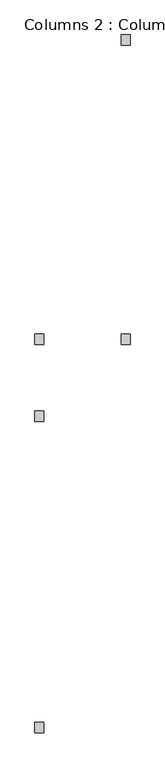
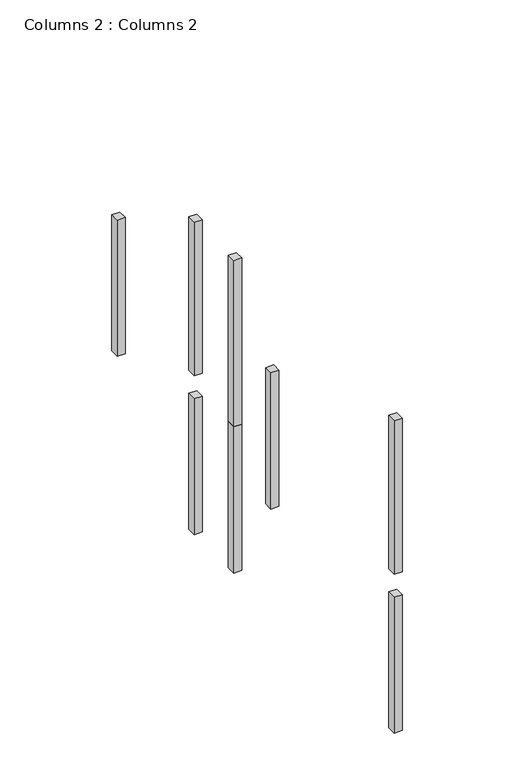
"""IFC4 building model written with IfcOpenShell, lengths in millimetres: column geometry, Columns 2 : Columns 2."""

from ifc_helpers import new_model, si_unit, frame, origin, place, context, project, spatial, polyline, outline, extrude, source, transform, mapped, element, save


def columns_2_columns_2_417d1360(model_context):
    return source(origin(), model_context, "Body", "SweptSolid", [
        extrude(outline(polyline([(31923.0340778, 35213.6207942), (31923.0340778, 35366.0207942), (32053.2090778, 35366.0207942), (32053.2090778, 35213.6207942), (31923.0340778, 35213.6207942)])), frame((0.0, 0.0, 268947.9), z_axis=(0.0, 0.0, 1.0), x_axis=(1.0, 0.0, 0.0)), (0.0, 0.0, 1.0), 2857.5),
        extrude(outline(polyline([(31923.0340778, 36331.2207942), (31923.0340778, 36483.6207942), (32053.2090778, 36483.6207942), (32053.2090778, 36331.2207942), (31923.0340778, 36331.2207942)])), frame((0.0, 0.0, 266414.25), z_axis=(0.0, 0.0, 1.0), x_axis=(1.0, 0.0, 0.0)), (0.0, 0.0, 1.0), 2335.2125),
        extrude(outline(polyline([(31923.0340778, 36331.2207942), (31923.0340778, 36483.6207942), (32053.2090778, 36483.6207942), (32053.2090778, 36331.2207942), (31923.0340778, 36331.2207942)])), frame((0.0, 0.0, 269146.3375), z_axis=(0.0, 0.0, 1.0), x_axis=(1.0, 0.0, 0.0)), (0.0, 0.0, 1.0), 2643.1875),
        extrude(outline(polyline([(31923.0340778, 35213.6207942), (31923.0340778, 35366.0207942), (32053.2090778, 35366.0207942), (32053.2090778, 35213.6207942), (31923.0340778, 35213.6207942)])), frame((0.0, 0.0, 266430.125), z_axis=(0.0, 0.0, 1.0), x_axis=(1.0, 0.0, 0.0)), (0.0, 0.0, 1.0), 2517.775),
        extrude(outline(polyline([(33172.4085525, 40668.9106612), (33172.4085525, 40821.3106612), (33302.5835525, 40821.3106612), (33302.5835525, 40668.9106612), (33172.4085525, 40668.9106612)])), frame((0.0, 0.0, 266414.25), z_axis=(0.0, 0.0, 1.0), x_axis=(1.0, 0.0, 0.0)), (0.0, 0.0, 1.0), 2343.15),
        extrude(outline(polyline([(33172.4085525, 36331.2207942), (33172.4085525, 36483.6207942), (33302.5835525, 36483.6207942), (33302.5835525, 36331.2207942), (33172.4085525, 36331.2207942)])), frame((0.0, 0.0, 266414.25), z_axis=(0.0, 0.0, 1.0), x_axis=(1.0, 0.0, 0.0)), (0.0, 0.0, 1.0), 2343.15),
        extrude(outline(polyline([(31923.0340778, 30698.1406612), (31923.0340778, 30850.5406612), (32053.2090778, 30850.5406612), (32053.2090778, 30698.1406612), (31923.0340778, 30698.1406612)])), frame((0.0, 0.0, 266414.25), z_axis=(0.0, 0.0, 1.0), x_axis=(1.0, 0.0, 0.0)), (0.0, 0.0, 1.0), 2335.2125),
        extrude(outline(polyline([(31923.0340778, 30698.1406612), (31923.0340778, 30850.5406612), (32053.2090778, 30850.5406612), (32053.2090778, 30698.1406612), (31923.0340778, 30698.1406612)])), frame((0.0, 0.0, 269146.3375), z_axis=(0.0, 0.0, 1.0), x_axis=(1.0, 0.0, 0.0)), (0.0, 0.0, 1.0), 2643.1875),
        extrude(outline(polyline([(31923.0340778, 30698.1406612), (31923.0340778, 30850.5406612), (32053.2090778, 30850.5406612), (32053.2090778, 30698.1406612), (31923.0340778, 30698.1406612)])), frame((0.0, 0.0, 266422.1875), z_axis=(0.0, 0.0, 1.0), x_axis=(1.0, 0.0, 0.0)), (0.0, 0.0, 1.0), 2327.275),
    ])


if __name__ == "__main__":
    model = new_model("IFC4")
    model_context = context("Model", 3, world=origin())
    ifc_project = project(units=[si_unit("LENGTHUNIT", "METRE", prefix="MILLI")], contexts=[model_context])
    site = spatial("IfcSite", under=ifc_project)
    building = spatial("IfcBuilding", under=site)
    placement = place(None, origin())
    columns_2_columns_2_shape = columns_2_columns_2_417d1360(model_context)
    element("IfcColumn", 1, ObjectType="Columns 2 : Columns 2", at=placement, inside=building, context=model_context, shape_type="MappedRepresentation", body=[
        mapped(columns_2_columns_2_shape, transform((0.0, 0.0, 0.0), x_axis=(1.0, 0.0, 0.0), y_axis=(0.0, 1.0, 0.0), z_axis=(0.0, 0.0, 1.0))),
    ])
    save(model, "model.ifc")

# Revit data of these elements
# Element 1 (IfcColumn, "Columns 2 : Columns 2")
#   Materials on its faces: "5 1/8\" x 6\" GLUELAM COLUMN"
# Materials
#   "5 1/8\" x 6\" GLUELAM COLUMN": class "Wood", colour RGB 144 113 62, transparency 0, Description = "Pinus Echinata", Cost = 0
